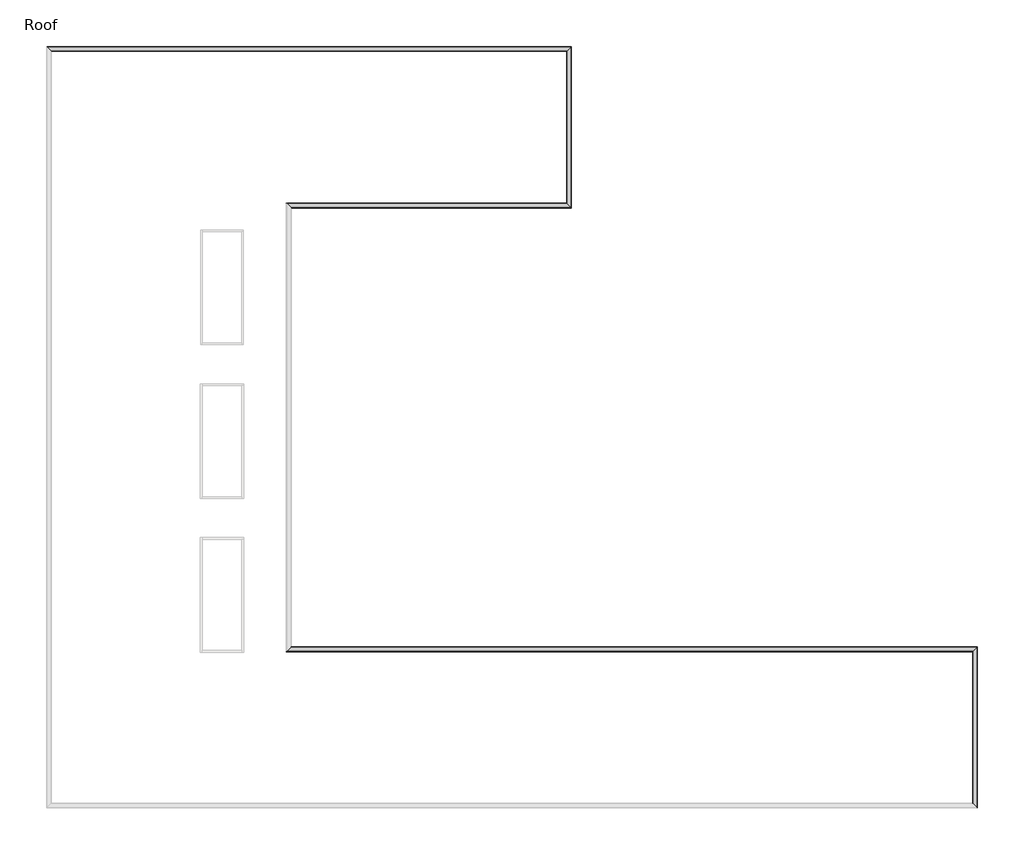
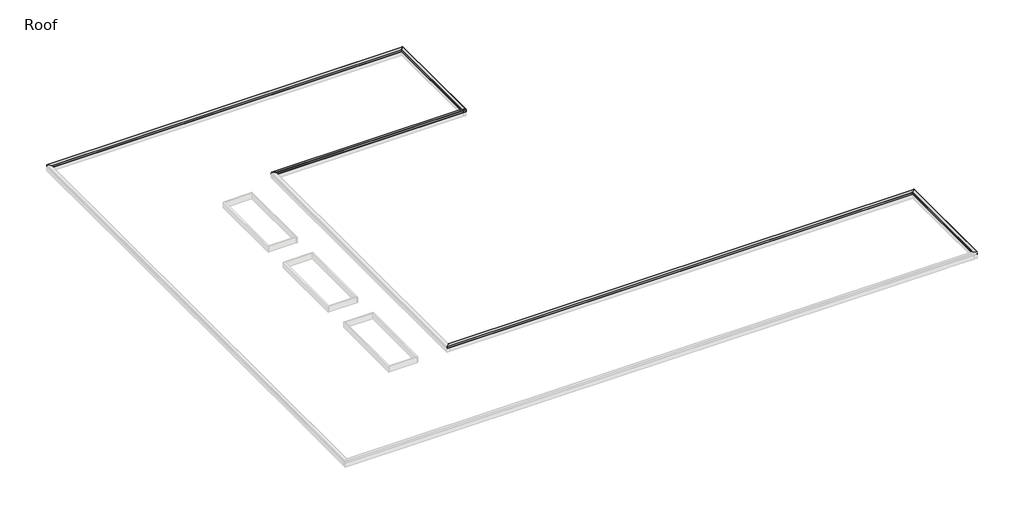
# One storey, part 2 of 2: 5 proxies.
"""IFC4 building model written with IfcOpenShell, lengths in millimetres."""

from ifc_helpers import new_model, si_unit, frame, origin, place, context, project, spatial, ellipse_curve, element, save
from ifc_brep_helpers import plane_surface, cylinder_surface, advanced_brep

model = new_model("IFC4")

# Units and contexts
model_context = context("Model", 3, world=origin())
ifc_project = project(units=[si_unit("LENGTHUNIT", "METRE", prefix="MILLI")], contexts=[model_context])

# Site, building, storey
site = spatial("IfcSite", under=ifc_project)
building = spatial("IfcBuilding", under=site)
storey = spatial("IfcBuildingStorey", under=building, Name="Roof", Elevation=10972.8)

# Proxies
placement = place(None, origin())
element("IfcBuildingElementProxy", 1, Name="Wall Sweeps", at=placement, inside=storey, context=model_context, shape_type="AdvancedBrep", body=[
    advanced_brep(
    [(37361.1457476, 54038.425, 11636.9329619), (37361.1457476, 54038.425, 11647.1824239), (37364.3207476, 54041.6, 11647.1824239), (37364.3207476, 54041.6, 11431.2824239), (37381.3349718, 54058.6142242, 11414.2681997), (37379.1062599, 54056.3855122, 11412.0394878), (37361.1457476, 54038.425, 11430.0), (37361.1457476, 54038.425, 11633.7462366), (37053.1707476, 53730.45, 11607.2537634), (37053.1707476, 53730.45, 11430.0), (37035.2102354, 53712.4894877, 11412.0394878), (37032.9651714, 53710.2444237, 11414.2845518), (37049.9957476, 53727.275, 11431.3151281), (37049.9957476, 53727.275, 11607.5268817), (37044.7672416, 53722.0464939, 11607.0771178), (37045.8777162, 53723.1569685, 11609.8131313), (37361.1457476, 42551.275, 11636.9329619), (37045.8777162, 42866.5430314, 11609.8131313), (37044.7672416, 42867.653506, 11607.0771178), (37049.9957476, 42862.425, 11607.5268817), (37049.9957476, 42862.425, 11431.3151281), (37032.9651714, 42879.4555762, 11414.2845518), (37035.2102354, 42877.2105122, 11412.0394878), (37053.1707476, 42859.25, 11430.0), (37053.1707476, 42859.25, 11607.2537634), (37361.1457476, 42551.275, 11633.7462366), (37361.1457476, 42551.275, 11430.0), (37379.1062599, 42533.3144877, 11412.0394878), (37381.3349718, 42531.0857758, 11414.2681997), (37364.3207476, 42548.1, 11431.2824239), (37364.3207476, 42548.1, 11647.1824239), (37361.1457476, 42551.275, 11647.1824239)],
    [
        (0, 1),
        (1, 2, ellipse_curve(frame((37362.7332476, 54040.0125, 11647.1824239), z_axis=(-0.7071067811865476, 0.7071067811865476, 0.0), x_axis=(0.7071067811865477, 0.7071067811865474, 0.0)), 2.245064, 1.5875)),
        (2, 3),
        (3, 4),
        (4, 5),
        (5, 6),
        (6, 7),
        (7, 8),
        (8, 9),
        (9, 10),
        (10, 11),
        (11, 12),
        (12, 13),
        (13, 14),
        (14, 15, ellipse_curve(frame((37044.7672416, 53722.0464939, 11608.6704804), z_axis=(-0.7071067811865476, 0.7071067811865476, 0.0), x_axis=(0.7071067811865477, 0.7071067811865474, 0.0)), 2.2533551, 1.5933627)),
        (15, 0),
        (16, 17),
        (17, 18, ellipse_curve(frame((37044.7672416, 42867.653506, 11608.6704804), z_axis=(-0.7071067811865547, -0.7071067811865405, 0.0), x_axis=(-0.7071067811865406, 0.7071067811865546, 0.0)), 2.2533551, 1.5933627)),
        (18, 19),
        (19, 20),
        (20, 21),
        (21, 22),
        (22, 23),
        (23, 24),
        (24, 25),
        (25, 26),
        (26, 27),
        (27, 28),
        (28, 29),
        (29, 30),
        (30, 31, ellipse_curve(frame((37362.7332476, 42549.6875, 11647.1824239), z_axis=(-0.7071067811865547, -0.7071067811865405, 0.0), x_axis=(-0.7071067811865406, 0.7071067811865546, 0.0)), 2.245064, 1.5875)),
        (31, 16),
        (0, 16),
        (31, 1),
        (30, 2),
        (29, 3),
        (28, 4),
        (27, 5),
        (26, 6),
        (25, 7),
        (24, 8),
        (23, 9),
        (22, 10),
        (21, 11),
        (20, 12),
        (19, 13),
        (18, 14),
        (17, 15),
    ],
    [
        plane_surface(frame((37354.7957476, 54032.075, 11887.2), z_axis=(-0.7071067811865476, 0.7071067811865476, 0.0), x_axis=(-0.7071067811865476, -0.7071067811865476, 0.0))),
        plane_surface(frame((37354.7957476, 42557.625, 11887.2), z_axis=(-0.7071067811865547, -0.7071067811865405, 0.0), x_axis=(-0.7071067811865405, 0.7071067811865547, 0.0))),
        plane_surface(frame((37361.1457476, 54038.425, 11636.9329619), z_axis=(-1.0, 0.0, 0.0), x_axis=(0.0, -1.0, 0.0))),
        cylinder_surface(frame((37362.7332476, 54032.075, 11647.1824239), z_axis=(0.0, 1.0, 0.0), x_axis=(-1.0, 0.0, 0.0)), 1.5875),
        plane_surface(frame((37364.3207476, 54041.6, 11647.1824239), z_axis=(1.0, 0.0, 0.0), x_axis=(0.0, -1.0, 0.0))),
        plane_surface(frame((37364.3207476, 54041.6, 11431.2824239), z_axis=(0.7071067811865493, 0.0, 0.7071067811865457), x_axis=(0.0, -1.0, 0.0))),
        plane_surface(frame((37381.3349718, 54058.6142242, 11414.2681997), z_axis=(0.7071067811865459, 0.0, -0.7071067811865492), x_axis=(0.0, -1.0, 0.0))),
        plane_surface(frame((37379.1062599, 54056.3855122, 11412.0394878), z_axis=(-0.7071067811865472, 0.0, -0.7071067811865478), x_axis=(0.0, -1.0, 0.0))),
        plane_surface(frame((37361.1457476, 54038.425, 11430.0), z_axis=(-1.0, 0.0, 0.0), x_axis=(0.0, -1.0, 0.0))),
        plane_surface(frame((37361.1457476, 54038.425, 11633.7462366), z_axis=(0.08570499422239307, 0.0, -0.9963205578353483), x_axis=(0.0, -1.0, 0.0))),
        plane_surface(frame((37053.1707476, 53730.45, 11607.2537634), z_axis=(1.0, 0.0, 0.0), x_axis=(0.0, -1.0, 0.0))),
        plane_surface(frame((37053.1707476, 53730.45, 11430.0), z_axis=(0.707106781186549, 0.0, -0.707106781186546), x_axis=(0.0, -1.0, 0.0))),
        plane_surface(frame((37035.2102354, 53712.4894877, 11412.0394878), z_axis=(-0.7071067811865422, 0.0, -0.7071067811865529), x_axis=(0.0, -1.0, 0.0))),
        plane_surface(frame((37032.9651714, 53710.2444237, 11414.2845518), z_axis=(-0.7071067811865496, 0.0, 0.7071067811865456), x_axis=(0.0, -1.0, 0.0))),
        plane_surface(frame((37049.9957476, 53727.275, 11431.3151281), z_axis=(-1.0, 0.0, 0.0), x_axis=(0.0, -1.0, 0.0))),
        plane_surface(frame((37049.9957476, 53727.275, 11607.5268817), z_axis=(0.08570499422239307, 0.0, -0.9963205578353483), x_axis=(0.0, -1.0, 0.0))),
        cylinder_surface(frame((37044.7672416, 54032.075, 11608.6704804), z_axis=(0.0, 1.0, 0.0), x_axis=(-1.0, 0.0, 0.0)), 1.5933627),
        plane_surface(frame((37045.8777162, 53723.1569685, 11609.8131313), z_axis=(-0.08570499422239307, 0.0, 0.9963205578353483), x_axis=(0.0, -1.0, 0.0))),
    ],
    [
        (0, [[1, 2, 3, 4, 5, 6, 7, 8, 9, 10, 11, 12, 13, 14, 15, 16]]),
        (1, [[17, 18, 19, 20, 21, 22, 23, 24, 25, 26, 27, 28, 29, 30, 31, 32]]),
        (2, [[-1, 33, -32, 34]]),
        (3, [[-2, -34, -31, 35]]),
        (4, [[-3, -35, -30, 36]]),
        (5, [[-4, -36, -29, 37]]),
        (6, [[-5, -37, -28, 38]]),
        (7, [[-6, -38, -27, 39]]),
        (8, [[-7, -39, -26, 40]]),
        (9, [[-8, -40, -25, 41]]),
        (10, [[-9, -41, -24, 42]]),
        (11, [[-10, -42, -23, 43]]),
        (12, [[-11, -43, -22, 44]]),
        (13, [[-12, -44, -21, 45]]),
        (14, [[-13, -45, -20, 46]]),
        (15, [[-14, -46, -19, 47]]),
        (16, [[-15, -47, -18, 48]]),
        (17, [[-16, -48, -17, -33]]),
    ],
),
])
element("IfcBuildingElementProxy", 2, Name="Wall Sweeps", at=placement, inside=storey, context=model_context, shape_type="AdvancedBrep", body=[
    advanced_brep(
    [(37361.1457476, 42551.275, 11636.9329619), (37361.1457476, 42551.275, 11647.1824239), (37364.3207476, 42548.1, 11647.1824239), (37364.3207476, 42548.1, 11431.2824239), (37381.3349718, 42531.0857758, 11414.2681997), (37379.1062599, 42533.3144877, 11412.0394878), (37361.1457476, 42551.275, 11430.0), (37361.1457476, 42551.275, 11633.7462366), (37053.1707476, 42859.25, 11607.2537634), (37053.1707476, 42859.25, 11430.0), (37035.2102354, 42877.2105122, 11412.0394878), (37032.9651714, 42879.4555762, 11414.2845518), (37049.9957476, 42862.425, 11431.3151281), (37049.9957476, 42862.425, 11607.5268817), (37044.7672416, 42867.653506, 11607.0771178), (37045.8777162, 42866.5430314, 11609.8131313), (17384.0457476, 42551.275, 11636.9329619), (17068.7777162, 42866.5430314, 11609.8131313), (17067.6672416, 42867.653506, 11607.0771178), (17072.8957476, 42862.425, 11607.5268817), (17072.8957476, 42862.425, 11431.3151281), (17055.8651714, 42879.4555762, 11414.2845518), (17058.1102354, 42877.2105122, 11412.0394878), (17076.0707476, 42859.25, 11430.0), (17076.0707476, 42859.25, 11607.2537634), (17384.0457476, 42551.275, 11633.7462366), (17384.0457476, 42551.275, 11430.0), (17402.0062599, 42533.3144877, 11412.0394878), (17404.2349718, 42531.0857758, 11414.2681997), (17387.2207476, 42548.1, 11431.2824239), (17387.2207476, 42548.1, 11647.1824239), (17384.0457476, 42551.275, 11647.1824239)],
    [
        (0, 1),
        (1, 2, ellipse_curve(frame((37362.7332476, 42549.6875, 11647.1824239), z_axis=(0.7071067811865547, 0.7071067811865405, 0.0), x_axis=(0.7071067811865404, -0.7071067811865548, 0.0)), 2.245064, 1.5875)),
        (2, 3),
        (3, 4),
        (4, 5),
        (5, 6),
        (6, 7),
        (7, 8),
        (8, 9),
        (9, 10),
        (10, 11),
        (11, 12),
        (12, 13),
        (13, 14),
        (14, 15, ellipse_curve(frame((37044.7672416, 42867.653506, 11608.6704804), z_axis=(0.7071067811865547, 0.7071067811865405, 0.0), x_axis=(0.7071067811865404, -0.7071067811865548, 0.0)), 2.2533551, 1.5933627)),
        (15, 0),
        (16, 17),
        (17, 18, ellipse_curve(frame((17067.6672416, 42867.653506, 11608.6704804), z_axis=(-0.7071067811865511, -0.707106781186544, 0.0), x_axis=(0.7071067811865439, -0.7071067811865511, 0.0)), 2.2533551, 1.5933627)),
        (18, 19),
        (19, 20),
        (20, 21),
        (21, 22),
        (22, 23),
        (23, 24),
        (24, 25),
        (25, 26),
        (26, 27),
        (27, 28),
        (28, 29),
        (29, 30),
        (30, 31, ellipse_curve(frame((17385.6332476, 42549.6875, 11647.1824239), z_axis=(-0.7071067811865511, -0.707106781186544, 0.0), x_axis=(0.7071067811865439, -0.7071067811865511, 0.0)), 2.245064, 1.5875)),
        (31, 16),
        (0, 16),
        (31, 1),
        (30, 2),
        (29, 3),
        (28, 4),
        (27, 5),
        (26, 6),
        (25, 7),
        (24, 8),
        (23, 9),
        (22, 10),
        (21, 11),
        (20, 12),
        (19, 13),
        (18, 14),
        (17, 15),
    ],
    [
        plane_surface(frame((37354.7957476, 42557.625, 11887.2), z_axis=(0.7071067811865547, 0.7071067811865405, 0.0), x_axis=(-0.7071067811865405, 0.7071067811865547, 0.0))),
        plane_surface(frame((17377.6957476, 42557.625, 11277.6), z_axis=(-0.7071067811865511, -0.707106781186544, 0.0), x_axis=(0.707106781186544, -0.7071067811865511, 0.0))),
        plane_surface(frame((37361.1457476, 42551.275, 11636.9329619), z_axis=(0.0, 1.0, 0.0), x_axis=(-1.0, 0.0, 0.0))),
        cylinder_surface(frame((37354.7957476, 42549.6875, 11647.1824239), z_axis=(1.0, 0.0, 0.0), x_axis=(0.0, 1.0, 0.0)), 1.5875),
        plane_surface(frame((37364.3207476, 42548.1, 11647.1824239), z_axis=(0.0, -1.0, 0.0), x_axis=(-1.0, 0.0, 0.0))),
        plane_surface(frame((37364.3207476, 42548.1, 11431.2824239), z_axis=(0.0, -0.7071067811865493, 0.7071067811865457), x_axis=(-1.0, 0.0, 0.0))),
        plane_surface(frame((37381.3349718, 42531.0857758, 11414.2681997), z_axis=(0.0, -0.7071067811865459, -0.7071067811865492), x_axis=(-1.0, 0.0, 0.0))),
        plane_surface(frame((37379.1062599, 42533.3144877, 11412.0394878), z_axis=(0.0, 0.7071067811865472, -0.7071067811865478), x_axis=(-1.0, 0.0, 0.0))),
        plane_surface(frame((37361.1457476, 42551.275, 11430.0), z_axis=(0.0, 1.0, 0.0), x_axis=(-1.0, 0.0, 0.0))),
        plane_surface(frame((37361.1457476, 42551.275, 11633.7462366), z_axis=(0.0, -0.08570499422239307, -0.9963205578353483), x_axis=(-1.0, 0.0, 0.0))),
        plane_surface(frame((37053.1707476, 42859.25, 11607.2537634), z_axis=(0.0, -1.0, 0.0), x_axis=(-1.0, 0.0, 0.0))),
        plane_surface(frame((37053.1707476, 42859.25, 11430.0), z_axis=(0.0, -0.707106781186549, -0.707106781186546), x_axis=(-1.0, 0.0, 0.0))),
        plane_surface(frame((37035.2102354, 42877.2105122, 11412.0394878), z_axis=(0.0, 0.7071067811865422, -0.7071067811865529), x_axis=(-1.0, 0.0, 0.0))),
        plane_surface(frame((37032.9651714, 42879.4555762, 11414.2845518), z_axis=(0.0, 0.7071067811865496, 0.7071067811865456), x_axis=(-1.0, 0.0, 0.0))),
        plane_surface(frame((37049.9957476, 42862.425, 11431.3151281), z_axis=(0.0, 1.0, 0.0), x_axis=(-1.0, 0.0, 0.0))),
        plane_surface(frame((37049.9957476, 42862.425, 11607.5268817), z_axis=(0.0, -0.08570499422239307, -0.9963205578353483), x_axis=(-1.0, 0.0, 0.0))),
        cylinder_surface(frame((37354.7957476, 42867.653506, 11608.6704804), z_axis=(1.0, 0.0, 0.0), x_axis=(0.0, 1.0, 0.0)), 1.5933627),
        plane_surface(frame((37045.8777162, 42866.5430314, 11609.8131313), z_axis=(0.0, 0.08570499422239307, 0.9963205578353483), x_axis=(-1.0, 0.0, 0.0))),
    ],
    [
        (0, [[1, 2, 3, 4, 5, 6, 7, 8, 9, 10, 11, 12, 13, 14, 15, 16]]),
        (1, [[17, 18, 19, 20, 21, 22, 23, 24, 25, 26, 27, 28, 29, 30, 31, 32]]),
        (2, [[-1, 33, -32, 34]]),
        (3, [[-2, -34, -31, 35]]),
        (4, [[-3, -35, -30, 36]]),
        (5, [[-4, -36, -29, 37]]),
        (6, [[-5, -37, -28, 38]]),
        (7, [[-6, -38, -27, 39]]),
        (8, [[-7, -39, -26, 40]]),
        (9, [[-8, -40, -25, 41]]),
        (10, [[-9, -41, -24, 42]]),
        (11, [[-10, -42, -23, 43]]),
        (12, [[-11, -43, -22, 44]]),
        (13, [[-12, -44, -21, 45]]),
        (14, [[-13, -45, -20, 46]]),
        (15, [[-14, -46, -19, 47]]),
        (16, [[-15, -47, -18, 48]]),
        (17, [[-16, -48, -17, -33]]),
    ],
),
])
element("IfcBuildingElementProxy", 3, Name="Wall Sweeps", at=placement, inside=storey, context=model_context, shape_type="AdvancedBrep", body=[
    advanced_brep(
    [(17384.0457476, 11201.325, 11636.9329619), (17384.0457476, 11201.325, 11647.1824239), (17387.2207476, 11204.5, 11647.1824239), (17387.2207476, 11204.5, 11431.2824239), (17404.2349718, 11221.5142242, 11414.2681997), (17402.0062599, 11219.2855122, 11412.0394878), (17384.0457476, 11201.325, 11430.0), (17384.0457476, 11201.325, 11633.7462366), (17076.0707476, 10893.35, 11607.2537634), (17076.0707476, 10893.35, 11430.0), (17058.1102354, 10875.3894877, 11412.0394878), (17055.8651714, 10873.1444237, 11414.2845518), (17072.8957476, 10890.175, 11431.3151281), (17072.8957476, 10890.175, 11607.5268817), (17067.6672416, 10884.9464939, 11607.0771178), (17068.7777162, 10886.0569685, 11609.8131313), (66317.1457476, 11201.325, 11636.9329619), (66001.8777162, 10886.0569685, 11609.8131313), (66000.7672416, 10884.9464939, 11607.0771178), (66005.9957476, 10890.175, 11607.5268817), (66005.9957476, 10890.175, 11431.3151281), (65988.9651714, 10873.1444237, 11414.2845518), (65991.2102354, 10875.3894877, 11412.0394878), (66009.1707476, 10893.35, 11430.0), (66009.1707476, 10893.35, 11607.2537634), (66317.1457476, 11201.325, 11633.7462366), (66317.1457476, 11201.325, 11430.0), (66335.1062599, 11219.2855122, 11412.0394878), (66337.3349718, 11221.5142242, 11414.2681997), (66320.3207476, 11204.5, 11431.2824239), (66320.3207476, 11204.5, 11647.1824239), (66317.1457476, 11201.325, 11647.1824239)],
    [
        (0, 1),
        (1, 2, ellipse_curve(frame((17385.6332476, 11202.9125, 11647.1824239), z_axis=(-0.7071067811865476, 0.7071067811865476, 0.0), x_axis=(-0.7071067811865475, -0.7071067811865476, 0.0)), 2.245064, 1.5875)),
        (2, 3),
        (3, 4),
        (4, 5),
        (5, 6),
        (6, 7),
        (7, 8),
        (8, 9),
        (9, 10),
        (10, 11),
        (11, 12),
        (12, 13),
        (13, 14),
        (14, 15, ellipse_curve(frame((17067.6672416, 10884.9464939, 11608.6704804), z_axis=(-0.7071067811865476, 0.7071067811865476, 0.0), x_axis=(-0.7071067811865475, -0.7071067811865476, 0.0)), 2.2533551, 1.5933627)),
        (15, 0),
        (16, 17),
        (17, 18, ellipse_curve(frame((66000.7672416, 10884.9464939, 11608.6704804), z_axis=(0.707106781186544, -0.7071067811865511, 0.0), x_axis=(-0.7071067811865509, -0.707106781186544, 0.0)), 2.2533551, 1.5933627)),
        (18, 19),
        (19, 20),
        (20, 21),
        (21, 22),
        (22, 23),
        (23, 24),
        (24, 25),
        (25, 26),
        (26, 27),
        (27, 28),
        (28, 29),
        (29, 30),
        (30, 31, ellipse_curve(frame((66318.7332476, 11202.9125, 11647.1824239), z_axis=(0.707106781186544, -0.7071067811865511, 0.0), x_axis=(-0.7071067811865509, -0.707106781186544, 0.0)), 2.245064, 1.5875)),
        (31, 16),
        (0, 16),
        (31, 1),
        (30, 2),
        (29, 3),
        (28, 4),
        (27, 5),
        (26, 6),
        (25, 7),
        (24, 8),
        (23, 9),
        (22, 10),
        (21, 11),
        (20, 12),
        (19, 13),
        (18, 14),
        (17, 15),
    ],
    [
        plane_surface(frame((17377.6957476, 11194.975, 11277.6), z_axis=(-0.7071067811865476, 0.7071067811865476, 0.0), x_axis=(0.7071067811865476, 0.7071067811865476, 0.0))),
        plane_surface(frame((66310.7957476, 11194.975, 11887.2), z_axis=(0.707106781186544, -0.7071067811865511, 0.0), x_axis=(-0.7071067811865511, -0.707106781186544, 0.0))),
        plane_surface(frame((17384.0457476, 11201.325, 11636.9329619), z_axis=(0.0, -1.0, 0.0), x_axis=(1.0, 0.0, 0.0))),
        cylinder_surface(frame((17377.6957476, 11202.9125, 11647.1824239), z_axis=(-1.0, 0.0, 0.0), x_axis=(0.0, -1.0, 0.0)), 1.5875),
        plane_surface(frame((17387.2207476, 11204.5, 11647.1824239), z_axis=(0.0, 1.0, 0.0), x_axis=(1.0, 0.0, 0.0))),
        plane_surface(frame((17387.2207476, 11204.5, 11431.2824239), z_axis=(0.0, 0.7071067811865493, 0.7071067811865457), x_axis=(1.0, 0.0, 0.0))),
        plane_surface(frame((17404.2349718, 11221.5142242, 11414.2681997), z_axis=(0.0, 0.7071067811865459, -0.7071067811865492), x_axis=(1.0, 0.0, 0.0))),
        plane_surface(frame((17402.0062599, 11219.2855122, 11412.0394878), z_axis=(0.0, -0.7071067811865472, -0.7071067811865478), x_axis=(1.0, 0.0, 0.0))),
        plane_surface(frame((17384.0457476, 11201.325, 11430.0), z_axis=(0.0, -1.0, 0.0), x_axis=(1.0, 0.0, 0.0))),
        plane_surface(frame((17384.0457476, 11201.325, 11633.7462366), z_axis=(0.0, 0.08570499422239307, -0.9963205578353483), x_axis=(1.0, 0.0, 0.0))),
        plane_surface(frame((17076.0707476, 10893.35, 11607.2537634), z_axis=(0.0, 1.0, 0.0), x_axis=(1.0, 0.0, 0.0))),
        plane_surface(frame((17076.0707476, 10893.35, 11430.0), z_axis=(0.0, 0.707106781186549, -0.707106781186546), x_axis=(1.0, 0.0, 0.0))),
        plane_surface(frame((17058.1102354, 10875.3894877, 11412.0394878), z_axis=(0.0, -0.7071067811865422, -0.7071067811865529), x_axis=(1.0, 0.0, 0.0))),
        plane_surface(frame((17055.8651714, 10873.1444237, 11414.2845518), z_axis=(0.0, -0.7071067811865496, 0.7071067811865456), x_axis=(1.0, 0.0, 0.0))),
        plane_surface(frame((17072.8957476, 10890.175, 11431.3151281), z_axis=(0.0, -1.0, 0.0), x_axis=(1.0, 0.0, 0.0))),
        plane_surface(frame((17072.8957476, 10890.175, 11607.5268817), z_axis=(0.0, 0.08570499422239307, -0.9963205578353483), x_axis=(1.0, 0.0, 0.0))),
        cylinder_surface(frame((17377.6957476, 10884.9464939, 11608.6704804), z_axis=(-1.0, 0.0, 0.0), x_axis=(0.0, -1.0, 0.0)), 1.5933627),
        plane_surface(frame((17068.7777162, 10886.0569685, 11609.8131313), z_axis=(0.0, -0.08570499422239307, 0.9963205578353483), x_axis=(1.0, 0.0, 0.0))),
    ],
    [
        (0, [[1, 2, 3, 4, 5, 6, 7, 8, 9, 10, 11, 12, 13, 14, 15, 16]]),
        (1, [[17, 18, 19, 20, 21, 22, 23, 24, 25, 26, 27, 28, 29, 30, 31, 32]]),
        (2, [[-1, 33, -32, 34]]),
        (3, [[-2, -34, -31, 35]]),
        (4, [[-3, -35, -30, 36]]),
        (5, [[-4, -36, -29, 37]]),
        (6, [[-5, -37, -28, 38]]),
        (7, [[-6, -38, -27, 39]]),
        (8, [[-7, -39, -26, 40]]),
        (9, [[-8, -40, -25, 41]]),
        (10, [[-9, -41, -24, 42]]),
        (11, [[-10, -42, -23, 43]]),
        (12, [[-11, -43, -22, 44]]),
        (13, [[-12, -44, -21, 45]]),
        (14, [[-13, -45, -20, 46]]),
        (15, [[-14, -46, -19, 47]]),
        (16, [[-15, -47, -18, 48]]),
        (17, [[-16, -48, -17, -33]]),
    ],
),
])
element("IfcBuildingElementProxy", 4, Name="Wall Sweeps", at=placement, inside=storey, context=model_context, shape_type="AdvancedBrep", body=[
    advanced_brep(
    [(66317.1457476, 11201.325, 11636.9329619), (66317.1457476, 11201.325, 11647.1824239), (66320.3207476, 11204.5, 11647.1824239), (66320.3207476, 11204.5, 11431.2824239), (66337.3349718, 11221.5142242, 11414.2681997), (66335.1062599, 11219.2855122, 11412.0394878), (66317.1457476, 11201.325, 11430.0), (66317.1457476, 11201.325, 11633.7462366), (66009.1707476, 10893.35, 11607.2537634), (66009.1707476, 10893.35, 11430.0), (65991.2102354, 10875.3894877, 11412.0394878), (65988.9651714, 10873.1444237, 11414.2845518), (66005.9957476, 10890.175, 11431.3151281), (66005.9957476, 10890.175, 11607.5268817), (66000.7672416, 10884.9464939, 11607.0771178), (66001.8777162, 10886.0569685, 11609.8131313), (66317.1457476, -260.425, 11636.9329619), (66001.8777162, 54.8430314, 11609.8131313), (66000.7672416, 55.953506, 11607.0771178), (66005.9957476, 50.725, 11607.5268817), (66005.9957476, 50.725, 11431.3151281), (65988.9651714, 67.7555762, 11414.2845518), (65991.2102354, 65.5105122, 11412.0394878), (66009.1707476, 47.55, 11430.0), (66009.1707476, 47.55, 11607.2537634), (66317.1457476, -260.425, 11633.7462366), (66317.1457476, -260.425, 11430.0), (66335.1062599, -278.3855123, 11412.0394878), (66337.3349718, -280.6142242, 11414.2681997), (66320.3207476, -263.6, 11431.2824239), (66320.3207476, -263.6, 11647.1824239), (66317.1457476, -260.425, 11647.1824239)],
    [
        (0, 1),
        (1, 2, ellipse_curve(frame((66318.7332476, 11202.9125, 11647.1824239), z_axis=(-0.707106781186544, 0.7071067811865511, 0.0), x_axis=(0.7071067811865511, 0.7071067811865438, 0.0)), 2.245064, 1.5875)),
        (2, 3),
        (3, 4),
        (4, 5),
        (5, 6),
        (6, 7),
        (7, 8),
        (8, 9),
        (9, 10),
        (10, 11),
        (11, 12),
        (12, 13),
        (13, 14),
        (14, 15, ellipse_curve(frame((66000.7672416, 10884.9464939, 11608.6704804), z_axis=(-0.707106781186544, 0.7071067811865511, 0.0), x_axis=(0.7071067811865511, 0.7071067811865438, 0.0)), 2.2533551, 1.5933627)),
        (15, 0),
        (16, 17),
        (17, 18, ellipse_curve(frame((66000.7672416, 55.953506, 11608.6704804), z_axis=(-0.7071067811865456, -0.7071067811865496, 0.0), x_axis=(-0.7071067811865496, 0.7071067811865454, 0.0)), 2.2533551, 1.5933627)),
        (18, 19),
        (19, 20),
        (20, 21),
        (21, 22),
        (22, 23),
        (23, 24),
        (24, 25),
        (25, 26),
        (26, 27),
        (27, 28),
        (28, 29),
        (29, 30),
        (30, 31, ellipse_curve(frame((66318.7332476, -262.0125, 11647.1824239), z_axis=(-0.7071067811865456, -0.7071067811865496, 0.0), x_axis=(-0.7071067811865496, 0.7071067811865454, 0.0)), 2.245064, 1.5875)),
        (31, 16),
        (0, 16),
        (31, 1),
        (30, 2),
        (29, 3),
        (28, 4),
        (27, 5),
        (26, 6),
        (25, 7),
        (24, 8),
        (23, 9),
        (22, 10),
        (21, 11),
        (20, 12),
        (19, 13),
        (18, 14),
        (17, 15),
    ],
    [
        plane_surface(frame((66310.7957476, 11194.975, 11887.2), z_axis=(-0.707106781186544, 0.7071067811865511, 0.0), x_axis=(-0.7071067811865511, -0.707106781186544, 0.0))),
        plane_surface(frame((66310.7957476, -254.075, 11887.2), z_axis=(-0.7071067811865456, -0.7071067811865496, 0.0), x_axis=(-0.7071067811865496, 0.7071067811865456, 0.0))),
        plane_surface(frame((66317.1457476, 11201.325, 11636.9329619), z_axis=(-1.0, 0.0, 0.0), x_axis=(0.0, -1.0, 0.0))),
        cylinder_surface(frame((66318.7332476, 11194.975, 11647.1824239), z_axis=(0.0, 1.0, 0.0), x_axis=(-1.0, 0.0, 0.0)), 1.5875),
        plane_surface(frame((66320.3207476, 11204.5, 11647.1824239), z_axis=(1.0, 0.0, 0.0), x_axis=(0.0, -1.0, 0.0))),
        plane_surface(frame((66320.3207476, 11204.5, 11431.2824239), z_axis=(0.7071067811865493, 0.0, 0.7071067811865457), x_axis=(0.0, -1.0, 0.0))),
        plane_surface(frame((66337.3349718, 11221.5142242, 11414.2681997), z_axis=(0.7071067811865459, 0.0, -0.7071067811865492), x_axis=(0.0, -1.0, 0.0))),
        plane_surface(frame((66335.1062599, 11219.2855122, 11412.0394878), z_axis=(-0.7071067811865472, 0.0, -0.7071067811865478), x_axis=(0.0, -1.0, 0.0))),
        plane_surface(frame((66317.1457476, 11201.325, 11430.0), z_axis=(-1.0, 0.0, 0.0), x_axis=(0.0, -1.0, 0.0))),
        plane_surface(frame((66317.1457476, 11201.325, 11633.7462366), z_axis=(0.08570499422239307, 0.0, -0.9963205578353483), x_axis=(0.0, -1.0, 0.0))),
        plane_surface(frame((66009.1707476, 10893.35, 11607.2537634), z_axis=(1.0, 0.0, 0.0), x_axis=(0.0, -1.0, 0.0))),
        plane_surface(frame((66009.1707476, 10893.35, 11430.0), z_axis=(0.707106781186549, 0.0, -0.707106781186546), x_axis=(0.0, -1.0, 0.0))),
        plane_surface(frame((65991.2102354, 10875.3894877, 11412.0394878), z_axis=(-0.7071067811865422, 0.0, -0.7071067811865529), x_axis=(0.0, -1.0, 0.0))),
        plane_surface(frame((65988.9651714, 10873.1444237, 11414.2845518), z_axis=(-0.7071067811865496, 0.0, 0.7071067811865456), x_axis=(0.0, -1.0, 0.0))),
        plane_surface(frame((66005.9957476, 10890.175, 11431.3151281), z_axis=(-1.0, 0.0, 0.0), x_axis=(0.0, -1.0, 0.0))),
        plane_surface(frame((66005.9957476, 10890.175, 11607.5268817), z_axis=(0.08570499422239307, 0.0, -0.9963205578353483), x_axis=(0.0, -1.0, 0.0))),
        cylinder_surface(frame((66000.7672416, 11194.975, 11608.6704804), z_axis=(0.0, 1.0, 0.0), x_axis=(-1.0, 0.0, 0.0)), 1.5933627),
        plane_surface(frame((66001.8777162, 10886.0569685, 11609.8131313), z_axis=(-0.08570499422239307, 0.0, 0.9963205578353483), x_axis=(0.0, -1.0, 0.0))),
    ],
    [
        (0, [[1, 2, 3, 4, 5, 6, 7, 8, 9, 10, 11, 12, 13, 14, 15, 16]]),
        (1, [[17, 18, 19, 20, 21, 22, 23, 24, 25, 26, 27, 28, 29, 30, 31, 32]]),
        (2, [[-1, 33, -32, 34]]),
        (3, [[-2, -34, -31, 35]]),
        (4, [[-3, -35, -30, 36]]),
        (5, [[-4, -36, -29, 37]]),
        (6, [[-5, -37, -28, 38]]),
        (7, [[-6, -38, -27, 39]]),
        (8, [[-7, -39, -26, 40]]),
        (9, [[-8, -40, -25, 41]]),
        (10, [[-9, -41, -24, 42]]),
        (11, [[-10, -42, -23, 43]]),
        (12, [[-11, -43, -22, 44]]),
        (13, [[-12, -44, -21, 45]]),
        (14, [[-13, -45, -20, 46]]),
        (15, [[-14, -46, -19, 47]]),
        (16, [[-15, -47, -18, 48]]),
        (17, [[-16, -48, -17, -33]]),
    ],
),
])
element("IfcBuildingElementProxy", 5, Name="Wall Sweeps", at=placement, inside=storey, context=model_context, shape_type="AdvancedBrep", body=[
    advanced_brep(
    [(-34.0042524, 54038.425, 11636.9329619), (-34.0042524, 54038.425, 11647.1824239), (-37.1792524, 54041.6, 11647.1824239), (-37.1792524, 54041.6, 11431.2824239), (-54.1934766, 54058.6142242, 11414.2681997), (-51.9647646, 54056.3855122, 11412.0394878), (-34.0042524, 54038.425, 11430.0), (-34.0042524, 54038.425, 11633.7462366), (273.9707476, 53730.45, 11607.2537634), (273.9707476, 53730.45, 11430.0), (291.9312599, 53712.4894877, 11412.0394878), (294.1763239, 53710.2444237, 11414.2845518), (277.1457476, 53727.275, 11431.3151281), (277.1457476, 53727.275, 11607.5268817), (282.3742537, 53722.0464939, 11607.0771178), (281.2637791, 53723.1569685, 11609.8131313), (37361.1457476, 54038.425, 11636.9329619), (37045.8777162, 53723.1569685, 11609.8131313), (37044.7672416, 53722.0464939, 11607.0771178), (37049.9957476, 53727.275, 11607.5268817), (37049.9957476, 53727.275, 11431.3151281), (37032.9651714, 53710.2444237, 11414.2845518), (37035.2102354, 53712.4894877, 11412.0394878), (37053.1707476, 53730.45, 11430.0), (37053.1707476, 53730.45, 11607.2537634), (37361.1457476, 54038.425, 11633.7462366), (37361.1457476, 54038.425, 11430.0), (37379.1062599, 54056.3855122, 11412.0394878), (37381.3349718, 54058.6142242, 11414.2681997), (37364.3207476, 54041.6, 11431.2824239), (37364.3207476, 54041.6, 11647.1824239), (37361.1457476, 54038.425, 11647.1824239)],
    [
        (0, 1),
        (1, 2, ellipse_curve(frame((-35.5917524, 54040.0125, 11647.1824239), z_axis=(-0.7071067811865507, -0.7071067811865445, 0.0), x_axis=(-0.7071067811865442, 0.7071067811865507, 0.0)), 2.245064, 1.5875)),
        (2, 3),
        (3, 4),
        (4, 5),
        (5, 6),
        (6, 7),
        (7, 8),
        (8, 9),
        (9, 10),
        (10, 11),
        (11, 12),
        (12, 13),
        (13, 14),
        (14, 15, ellipse_curve(frame((282.3742537, 53722.0464939, 11608.6704804), z_axis=(-0.7071067811865507, -0.7071067811865445, 0.0), x_axis=(-0.7071067811865442, 0.7071067811865507, 0.0)), 2.2533551, 1.5933627)),
        (15, 0),
        (16, 17),
        (17, 18, ellipse_curve(frame((37044.7672416, 53722.0464939, 11608.6704804), z_axis=(0.7071067811865476, -0.7071067811865476, 0.0), x_axis=(-0.7071067811865474, -0.7071067811865476, 0.0)), 2.2533551, 1.5933627)),
        (18, 19),
        (19, 20),
        (20, 21),
        (21, 22),
        (22, 23),
        (23, 24),
        (24, 25),
        (25, 26),
        (26, 27),
        (27, 28),
        (28, 29),
        (29, 30),
        (30, 31, ellipse_curve(frame((37362.7332476, 54040.0125, 11647.1824239), z_axis=(0.7071067811865476, -0.7071067811865476, 0.0), x_axis=(-0.7071067811865474, -0.7071067811865476, 0.0)), 2.245064, 1.5875)),
        (31, 16),
        (0, 16),
        (31, 1),
        (30, 2),
        (29, 3),
        (28, 4),
        (27, 5),
        (26, 6),
        (25, 7),
        (24, 8),
        (23, 9),
        (22, 10),
        (21, 11),
        (20, 12),
        (19, 13),
        (18, 14),
        (17, 15),
    ],
    [
        plane_surface(frame((-27.6542524, 54032.075, 11887.2), z_axis=(-0.7071067811865507, -0.7071067811865445, 0.0), x_axis=(0.7071067811865445, -0.7071067811865507, 0.0))),
        plane_surface(frame((37354.7957476, 54032.075, 11887.2), z_axis=(0.7071067811865476, -0.7071067811865476, 0.0), x_axis=(-0.7071067811865476, -0.7071067811865476, 0.0))),
        plane_surface(frame((-34.0042524, 54038.425, 11636.9329619), z_axis=(0.0, -1.0, 0.0), x_axis=(1.0, 0.0, 0.0))),
        cylinder_surface(frame((-27.6542524, 54040.0125, 11647.1824239), z_axis=(-1.0, 0.0, 0.0), x_axis=(0.0, -1.0, 0.0)), 1.5875),
        plane_surface(frame((-37.1792524, 54041.6, 11647.1824239), z_axis=(0.0, 1.0, 0.0), x_axis=(1.0, 0.0, 0.0))),
        plane_surface(frame((-37.1792524, 54041.6, 11431.2824239), z_axis=(0.0, 0.7071067811865493, 0.7071067811865457), x_axis=(1.0, 0.0, 0.0))),
        plane_surface(frame((-54.1934766, 54058.6142242, 11414.2681997), z_axis=(0.0, 0.7071067811865459, -0.7071067811865492), x_axis=(1.0, 0.0, 0.0))),
        plane_surface(frame((-51.9647646, 54056.3855122, 11412.0394878), z_axis=(0.0, -0.7071067811865472, -0.7071067811865478), x_axis=(1.0, 0.0, 0.0))),
        plane_surface(frame((-34.0042524, 54038.425, 11430.0), z_axis=(0.0, -1.0, 0.0), x_axis=(1.0, 0.0, 0.0))),
        plane_surface(frame((-34.0042524, 54038.425, 11633.7462366), z_axis=(0.0, 0.08570499422239307, -0.9963205578353483), x_axis=(1.0, 0.0, 0.0))),
        plane_surface(frame((273.9707476, 53730.45, 11607.2537634), z_axis=(0.0, 1.0, 0.0), x_axis=(1.0, 0.0, 0.0))),
        plane_surface(frame((273.9707476, 53730.45, 11430.0), z_axis=(0.0, 0.707106781186549, -0.707106781186546), x_axis=(1.0, 0.0, 0.0))),
        plane_surface(frame((291.9312599, 53712.4894877, 11412.0394878), z_axis=(0.0, -0.7071067811865422, -0.7071067811865529), x_axis=(1.0, 0.0, 0.0))),
        plane_surface(frame((294.1763239, 53710.2444237, 11414.2845518), z_axis=(0.0, -0.7071067811865496, 0.7071067811865456), x_axis=(1.0, 0.0, 0.0))),
        plane_surface(frame((277.1457476, 53727.275, 11431.3151281), z_axis=(0.0, -1.0, 0.0), x_axis=(1.0, 0.0, 0.0))),
        plane_surface(frame((277.1457476, 53727.275, 11607.5268817), z_axis=(0.0, 0.08570499422239307, -0.9963205578353483), x_axis=(1.0, 0.0, 0.0))),
        cylinder_surface(frame((-27.6542524, 53722.0464939, 11608.6704804), z_axis=(-1.0, 0.0, 0.0), x_axis=(0.0, -1.0, 0.0)), 1.5933627),
        plane_surface(frame((281.2637791, 53723.1569685, 11609.8131313), z_axis=(0.0, -0.08570499422239307, 0.9963205578353483), x_axis=(1.0, 0.0, 0.0))),
    ],
    [
        (0, [[1, 2, 3, 4, 5, 6, 7, 8, 9, 10, 11, 12, 13, 14, 15, 16]]),
        (1, [[17, 18, 19, 20, 21, 22, 23, 24, 25, 26, 27, 28, 29, 30, 31, 32]]),
        (2, [[-1, 33, -32, 34]]),
        (3, [[-2, -34, -31, 35]]),
        (4, [[-3, -35, -30, 36]]),
        (5, [[-4, -36, -29, 37]]),
        (6, [[-5, -37, -28, 38]]),
        (7, [[-6, -38, -27, 39]]),
        (8, [[-7, -39, -26, 40]]),
        (9, [[-8, -40, -25, 41]]),
        (10, [[-9, -41, -24, 42]]),
        (11, [[-10, -42, -23, 43]]),
        (12, [[-11, -43, -22, 44]]),
        (13, [[-12, -44, -21, 45]]),
        (14, [[-13, -45, -20, 46]]),
        (15, [[-14, -46, -19, 47]]),
        (16, [[-15, -47, -18, 48]]),
        (17, [[-16, -48, -17, -33]]),
    ],
),
])

save(model, "model.ifc")

# Revit data of these elements
# Elements 1, 2, 3, 4, 5 (IfcBuildingElementProxy)
#   Phase Created = New Construction
#   Materials on its faces: "Metal - Aluminum"
# Materials
#   "Metal - Aluminum": class "Metal", colour RGB 140 140 140, transparency 0
